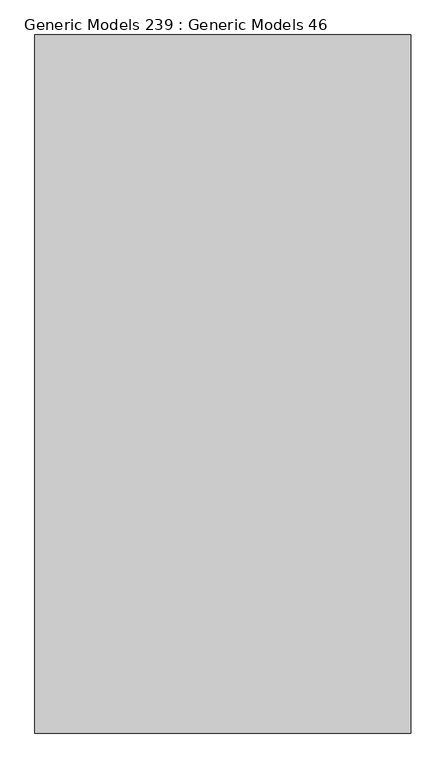
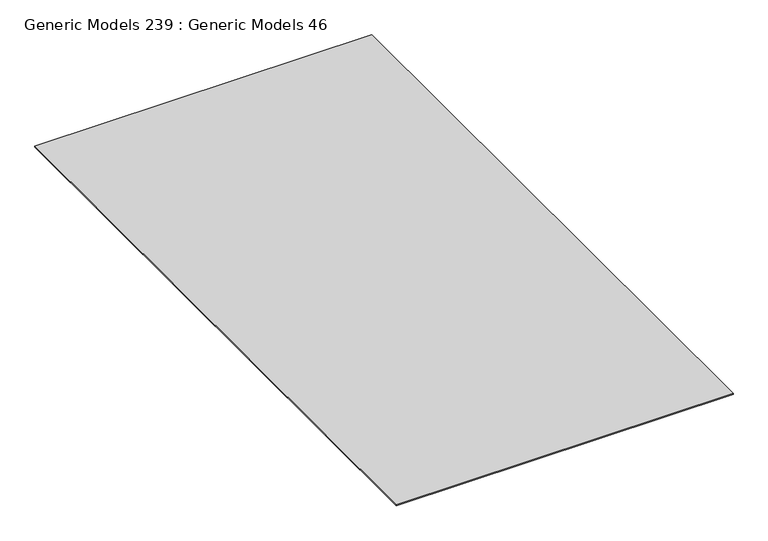
"""IFC4 building model written with IfcOpenShell, lengths in millimetres: proxy geometry, Generic Models 239 : Generic Models 46."""

from ifc_helpers import new_model, si_unit, frame, origin, place, context, project, spatial, polyline, outline, extrude, source, transform, mapped, element, save


def generic_models_239_generic_models_46_95e6735a(model_context):
    return source(origin(), model_context, "Body", "SweptSolid", [
        extrude(outline(polyline([(50347.5625, 0.0), (49691.4320511, 0.0), (49691.4320511, 1219.2), (50347.5625, 1219.2), (50347.5625, 0.0)])), frame((0.0, 0.0, 5505.7509163), z_axis=(0.0, 0.0, 1.0), x_axis=(1.0, 0.0, 0.0)), (0.0, 0.0, 1.0), 1.5875),
    ])


if __name__ == "__main__":
    model = new_model("IFC4")
    model_context = context("Model", 3, world=origin())
    ifc_project = project(units=[si_unit("LENGTHUNIT", "METRE", prefix="MILLI")], contexts=[model_context])
    site = spatial("IfcSite", under=ifc_project)
    building = spatial("IfcBuilding", under=site)
    placement = place(None, origin())
    generic_models_239_generic_models_46_shape = generic_models_239_generic_models_46_95e6735a(model_context)
    element("IfcBuildingElementProxy", 1, Name="Generic Models 239 : Generic Models 46", ObjectType="Generic Models 239 : Generic Models 46", at=placement, inside=building, context=model_context, shape_type="MappedRepresentation", body=[
        mapped(generic_models_239_generic_models_46_shape, transform((0.0, 0.0, 0.0), x_axis=(1.0, 0.0, 0.0), y_axis=(0.0, 1.0, 0.0), z_axis=(0.0, 0.0, 1.0))),
    ])
    save(model, "model.ifc")

# Revit data of these elements
# Element 1 (IfcBuildingElementProxy, "Generic Models 239 : Generic Models 46")
#   Materials on its faces: "SET IN BED OF SEALANT"
# Materials
#   "SET IN BED OF SEALANT": class "Unassigned", colour RGB 58 208 21, transparency 0, Cost = 0
